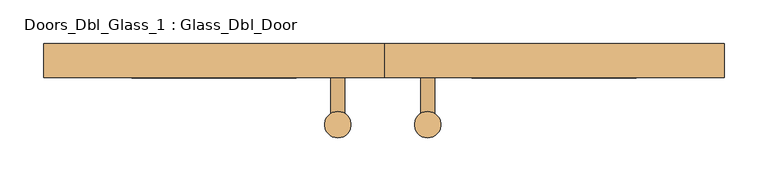
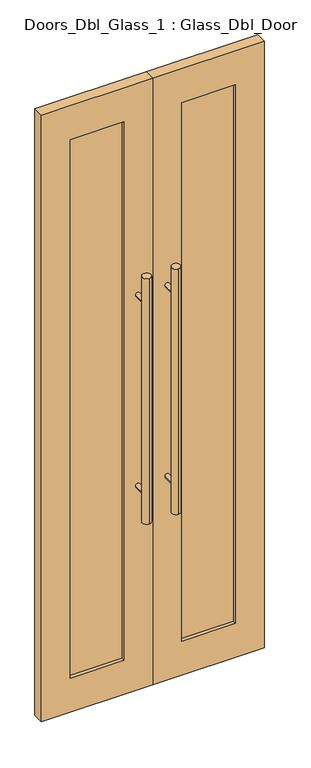
"""IFC4 building model written with IfcOpenShell, lengths in millimetres: door geometry, Doors_Dbl_Glass_1 : Glass_Dbl_Door."""

from ifc_helpers import new_model, si_unit, point, frame, frame_2d, origin, place, context, project, spatial, polyline, circle_curve, trimmed, segment, composite_curve, outline, extrude, source, transform, mapped, element, save


def doors_dbl_glass_1_glass_dbl_door_a30122f7(model_context):
    return source(origin(), model_context, "Body", "SweptSolid", [
        extrude(outline(composite_curve([segment(trimmed(circle_curve(frame_2d((49.6069979, -116.0715804)), 15.0), [point((49.6069979, -101.0715804))], [point((49.6069979, -131.0715804))], False, "CARTESIAN"), True, "CONTINUOUS"), segment(trimmed(circle_curve(frame_2d((49.6069979, -116.0715804)), 15.0), [point((49.6069979, -131.0715804))], [point((49.6069979, -101.0715804))], False, "CARTESIAN"), True, "CONTINUOUS")], self_intersect=False)), frame((0.0, 0.0, 650.0), z_axis=(0.0, 0.0, 1.0), x_axis=(1.0, 0.0, 0.0)), (0.0, 0.0, 1.0), 900.0),
        extrude(outline(composite_curve([segment(trimmed(circle_curve(frame_2d((-52.537897, -116.0715804)), 15.0), [point((-52.537897, -101.0715804))], [point((-52.537897, -131.0715804))], False, "CARTESIAN"), True, "CONTINUOUS"), segment(trimmed(circle_curve(frame_2d((-52.537897, -116.0715804)), 15.0), [point((-52.537897, -131.0715804))], [point((-52.537897, -101.0715804))], False, "CARTESIAN"), True, "CONTINUOUS")], self_intersect=False)), frame((0.0, 0.0, 650.0), z_axis=(0.0, 0.0, 1.0), x_axis=(1.0, 0.0, 0.0)), (0.0, 0.0, 1.0), 900.0),
        extrude(outline(composite_curve([segment(trimmed(circle_curve(frame_2d((750.0, 49.6069979)), 8.0), [point((750.0, 57.6069979))], [point((750.0, 41.6069979))], False, "CARTESIAN"), True, "CONTINUOUS"), segment(trimmed(circle_curve(frame_2d((750.0, 49.6069979)), 8.0), [point((750.0, 41.6069979))], [point((750.0, 57.6069979))], False, "CARTESIAN"), True, "CONTINUOUS")], self_intersect=False)), frame((0.0, -116.0715804, 0.0), z_axis=(0.0, 1.0, 0.0), x_axis=(0.0, 0.0, 1.0)), (0.0, 0.0, 1.0), 53.4927248),
        extrude(outline(composite_curve([segment(trimmed(circle_curve(frame_2d((750.0, -52.537897)), 8.0), [point((750.0, -44.537897))], [point((750.0, -60.537897))], False, "CARTESIAN"), True, "CONTINUOUS"), segment(trimmed(circle_curve(frame_2d((750.0, -52.537897)), 8.0), [point((750.0, -60.537897))], [point((750.0, -44.537897))], False, "CARTESIAN"), True, "CONTINUOUS")], self_intersect=False)), frame((0.0, -116.0715804, 0.0), z_axis=(0.0, 1.0, 0.0), x_axis=(0.0, 0.0, 1.0)), (0.0, 0.0, 1.0), 53.4927248),
        extrude(outline(composite_curve([segment(trimmed(circle_curve(frame_2d((1450.0, 49.6069979)), 8.0), [point((1450.0, 57.6069979))], [point((1450.0, 41.6069979))], False, "CARTESIAN"), True, "CONTINUOUS"), segment(trimmed(circle_curve(frame_2d((1450.0, 49.6069979)), 8.0), [point((1450.0, 41.6069979))], [point((1450.0, 57.6069979))], False, "CARTESIAN"), True, "CONTINUOUS")], self_intersect=False)), frame((0.0, -116.0715804, 0.0), z_axis=(0.0, 1.0, 0.0), x_axis=(0.0, 0.0, 1.0)), (0.0, 0.0, 1.0), 53.4927248),
        extrude(outline(composite_curve([segment(trimmed(circle_curve(frame_2d((1450.0, -52.537897)), 8.0), [point((1450.0, -44.537897))], [point((1450.0, -60.537897))], False, "CARTESIAN"), True, "CONTINUOUS"), segment(trimmed(circle_curve(frame_2d((1450.0, -52.537897)), 8.0), [point((1450.0, -60.537897))], [point((1450.0, -44.537897))], False, "CARTESIAN"), True, "CONTINUOUS")], self_intersect=False)), frame((0.0, -116.0715804, 0.0), z_axis=(0.0, 1.0, 0.0), x_axis=(0.0, 0.0, 1.0)), (0.0, 0.0, 1.0), 53.4927248),
        extrude(outline(polyline([(2225.0, -386.7001888), (0.0, -386.7001888), (0.0, 0.0), (2225.0, 0.0), (2225.0, -386.7001888)]), holes=[polyline([(2100.0, -286.7001888), (2100.0, -100.0), (125.0, -100.0), (125.0, -286.7001888), (2100.0, -286.7001888)])]), frame((0.0, -62.5788556, 0.0), z_axis=(0.0, 1.0, 0.0), x_axis=(0.0, 0.0, 1.0)), (0.0, 0.0, 1.0), 38.5435966),
        extrude(outline(polyline([(2225.0, 0.0), (0.0, 0.0), (0.0, 386.7001888), (2225.0, 386.7001888), (2225.0, 0.0)]), holes=[polyline([(2100.0, 100.0), (2100.0, 286.7001888), (125.0, 286.7001888), (125.0, 100.0), (2100.0, 100.0)])]), frame((0.0, -62.5788556, 0.0), z_axis=(0.0, 1.0, 0.0), x_axis=(0.0, 0.0, 1.0)), (0.0, 0.0, 1.0), 38.5435966),
        extrude(outline(polyline([(-100.0, -38.0), (-100.0, -50.0), (-286.7001888, -50.0), (-286.7001888, -38.0), (-100.0, -38.0)])), frame((0.0, 0.0, 125.0), z_axis=(0.0, 0.0, 1.0), x_axis=(1.0, 0.0, 0.0)), (0.0, 0.0, 1.0), 1975.0),
        extrude(outline(polyline([(286.7001888, -38.0), (286.7001888, -50.0), (100.0, -50.0), (100.0, -38.0), (286.7001888, -38.0)])), frame((0.0, 0.0, 125.0), z_axis=(0.0, 0.0, 1.0), x_axis=(1.0, 0.0, 0.0)), (0.0, 0.0, 1.0), 1975.0),
    ])


if __name__ == "__main__":
    model = new_model("IFC4")
    model_context = context("Model", 3, world=origin())
    ifc_project = project(units=[si_unit("LENGTHUNIT", "METRE", prefix="MILLI")], contexts=[model_context])
    site = spatial("IfcSite", under=ifc_project)
    building = spatial("IfcBuilding", under=site)
    placement = place(None, origin())
    doors_dbl_glass_1_glass_dbl_door_shape = doors_dbl_glass_1_glass_dbl_door_a30122f7(model_context)
    element("IfcDoor", 1, ObjectType="Doors_Dbl_Glass_1 : Glass_Dbl_Door", at=placement, inside=building, context=model_context, shape_type="MappedRepresentation", body=[
        mapped(doors_dbl_glass_1_glass_dbl_door_shape, transform((0.0, 0.0, 0.0), x_axis=(1.0, 0.0, 0.0), y_axis=(0.0, 1.0, 0.0), z_axis=(0.0, 0.0, 1.0))),
    ])
    save(model, "model.ifc")

# Revit data of these elements
# Type "Doors_Dbl_Glass_1 : Glass_Dbl_Door"
#   Type Mark = "47"
#   Construction Type Id = "GSP4R"
#   Analytic Construction = "1/8 in Pilkington single glazing"
#   Visual Light Transmittance = 0.9
#   Stile Shutting = 100 mm
#   Stile Hanging = 100 mm
#   Stile - Top Rail = 125 mm
#   Stile - Bottom Rail = 125 mm
#   Solar Heat Gain Coefficient = 0.78
#   Offset = 50 mm
#   Heat Transfer Coefficient (U) = 3.6886 W/(m²·K)
#   Glass Thickness = 12 mm
#   Define Thermal Properties by = 1
#   Material Ironmongery = Metal - Aluminum
#   Material Door = Metal - Aluminum
#   Material Glass = Glass
#   Function = (empty or 0)
# Element 1 (IfcDoor, "Doors_Dbl_Glass_1 : Glass_Dbl_Door")
#   Materials on its faces: "Metal - Aluminum", "Glass"
# Materials
#   "Metal - Aluminum": class "Metal", colour RGB 247 247 247, transparency 0
#   "Glass": class "Glass", colour RGB 0 128 192, transparency 0.9, Description = "Soda Lime Glass", Cost = 0
